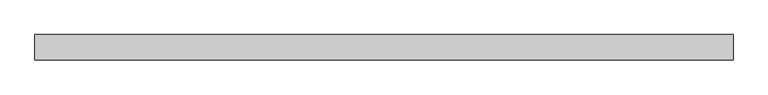
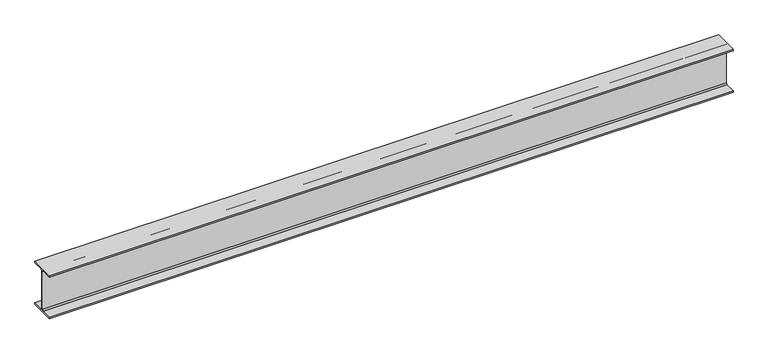
"""IFC4 building model written with IfcOpenShell, lengths in millimetres: beam geometry, Old_Steel Beam_H-KSD3502 : H_SB_ASB_H-482×300x11x15."""

from ifc_helpers import new_model, si_unit, point, frame, frame_2d, origin, place, context, project, spatial, polyline, circle_curve, trimmed, segment, composite_curve, outline, extrude, source, transform, mapped, element, save


def beam_863c03c5(model_context):
    return source(origin(), model_context, "Body", "SweptSolid", [
        extrude(outline(composite_curve([segment(polyline([(82.5, -141.5), (82.5, -151.7), (-82.5, -151.7), (-82.5, -141.5), (-11.9, -141.5)]), True, "CONTINUOUS"), segment(trimmed(circle_curve(frame_2d((-11.9, -132.6)), 8.9), [point((-11.9, -141.5))], [point((-3.0, -132.6))], True, "CARTESIAN"), True, "CONTINUOUS"), segment(polyline([(-3.0, -132.6), (-3.0, 132.6)]), True, "CONTINUOUS"), segment(trimmed(circle_curve(frame_2d((-11.9, 132.6)), 8.9), [point((-3.0, 132.6))], [point((-11.9, 141.5))], True, "CARTESIAN"), True, "CONTINUOUS"), segment(polyline([(-11.9, 141.5), (-82.5, 141.5), (-82.5, 151.7), (82.5, 151.7), (82.5, 141.5), (11.9, 141.5)]), True, "CONTINUOUS"), segment(trimmed(circle_curve(frame_2d((11.9, 132.6)), 8.9), [point((11.9, 141.5))], [point((3.0, 132.6))], True, "CARTESIAN"), True, "CONTINUOUS"), segment(polyline([(3.0, 132.6), (3.0, -132.6)]), True, "CONTINUOUS"), segment(trimmed(circle_curve(frame_2d((11.9, -132.6)), 8.9), [point((3.0, -132.6))], [point((11.9, -141.5))], True, "CARTESIAN"), True, "CONTINUOUS"), segment(polyline([(11.9, -141.5), (82.5, -141.5)]), True, "CONTINUOUS")], self_intersect=False)), frame((-2279.8, 0.0, 0.0), z_axis=(1.0, 0.0, 0.0), x_axis=(0.0, 1.0, 0.0)), (0.0, 0.0, 1.0), 4559.6),
    ])


if __name__ == "__main__":
    model = new_model("IFC4")
    model_context = context("Model", 3, world=origin())
    ifc_project = project(units=[si_unit("LENGTHUNIT", "METRE", prefix="MILLI")], contexts=[model_context])
    site = spatial("IfcSite", under=ifc_project)
    building = spatial("IfcBuilding", under=site)
    placement = place(None, origin())
    beam_shape = beam_863c03c5(model_context)
    element("IfcBeam", 1, ObjectType="Old_Steel Beam_H-KSD3502 : H_SB_ASB_H-482×300x11x15", at=placement, inside=building, context=model_context, shape_type="MappedRepresentation", body=[
        mapped(beam_shape, transform((0.0, 0.0, 0.0), x_axis=(1.0, 0.0, 0.0), y_axis=(0.0, 1.0, 0.0), z_axis=(0.0, 0.0, 1.0))),
    ])
    save(model, "model.ifc")

# Revit data of these elements
# Type "Old_Steel Beam_H-KSD3502 : H_SB_ASB_H-482×300x11x15"
#   Width = 30.0 cm
#   Web Thickness = 1.1 cm
#   Web Fillet = 2.6 cm
#   Warping Constant = 3680250.0 cm⁶
#   Torsional Moment of Inertia = 88.2192 cm⁴
#   Torsional Modulus = 1.0 cm³
#   Section Area = 145.5 cm²
#   Plastic Modulus weak axis = 695.0 cm³
#   Plastic Modulus strong axis = 2790.0 cm³
#   Perimeter = 2.10 m²/m
#   Nominal Weight = 114.00 kgf/m
#   Moment of Inertia weak axis = 6760.00 cm⁴
#   Moment of Inertia strong axis = 60400.00 cm⁴
#   Height = 48.2 cm
#   Flange Thickness = 1.5 cm
#   Elastic Modulus weak axis = 451.0 cm³
#   Elastic Modulus strong axis = 2500.0 cm³
#   Centroid Vertical = 24.1 cm
#   Centroid Horizontal = 15.0 cm
#   Length [instance default] = 1.5240 m
#   Structural Material [instance default] = Steel, 45-345
#   Assembly Code = ""
# Element 1 (IfcBeam, "Old_Steel Beam_H-KSD3502 : H_SB_ASB_H-482×300x11x15")
#   Structural Material = none
# Materials
#   "Steel, 45-345": class "Metal", colour RGB 189 187 185, transparency 0, Description = "Steel 345 MPa", Cost = 0
